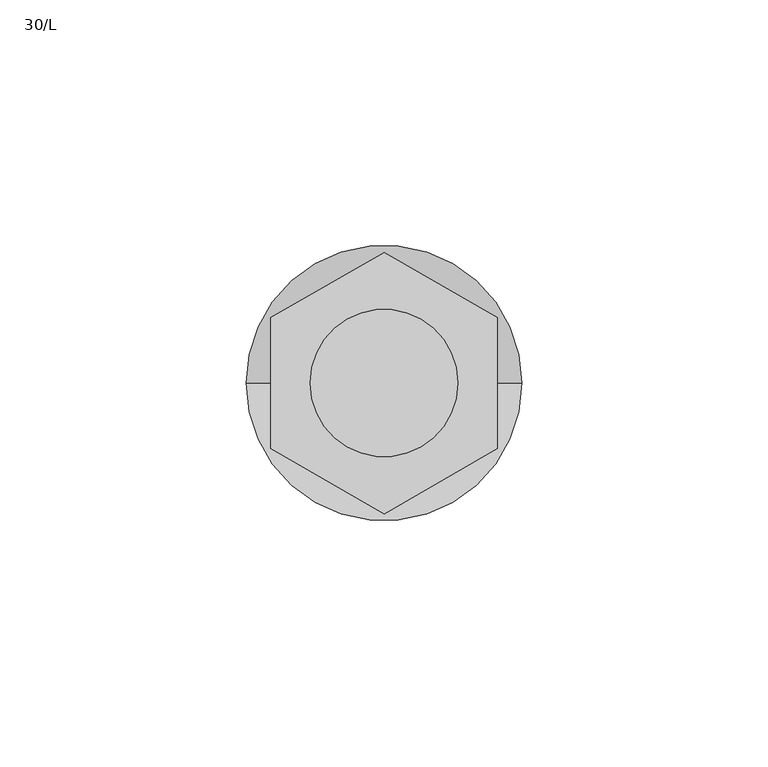
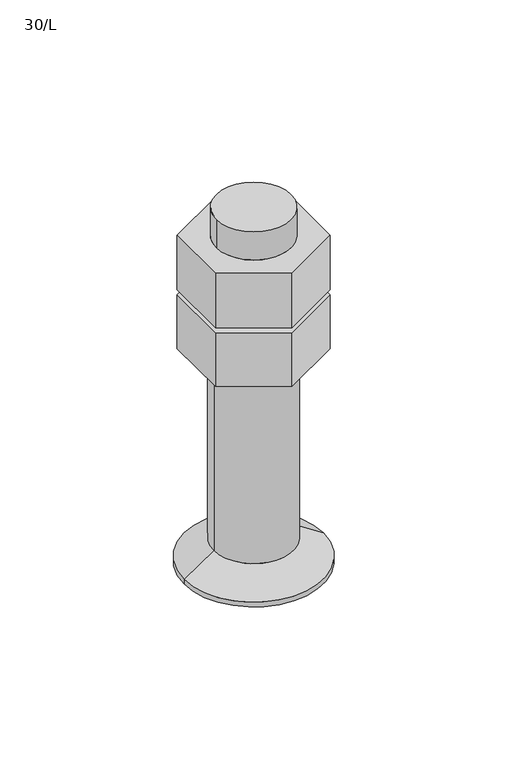
"""IFC4 building model written with IfcOpenShell, lengths in millimetres: fastener geometry, Bolt HPM-L : 30/L."""

from ifc_helpers import new_model, si_unit, frame, origin, origin_with_axes, place, context, project, spatial, polyline, circle_curve, source, transform, mapped, element, save
from ifc_brep_helpers import plane_surface, cylinder_surface, revolved_surface, advanced_brep


def fastener_30_l_d0df7ee6(model_context):
    return source(origin(), model_context, "Body", "AdvancedBrep", [
        advanced_brep(
        [(-23.0, -13.2790562, 22.7), (0.0, -26.5581124, 22.7), (23.0, -13.2790562, 22.7), (23.0, 13.2790562, 22.7), (0.0, 26.5581124, 22.7), (-23.0, 13.2790562, 22.7), (15.0, 0.0, 22.7), (-15.0, 0.0, 22.7), (-23.0, 13.2790562, 0.0), (-23.0, -13.2790562, 0.0), (0.0, 26.5581124, 0.0), (23.0, 13.2790562, 0.0), (23.0, -13.2790562, 0.0), (0.0, -26.5581124, 0.0), (-15.0, 0.0, 60.0), (15.0, 0.0, 60.0), (15.0, 0.0, 48.0), (-15.0, 0.0, 48.0), (-15.0, 0.0, 25.0), (15.0, 0.0, 25.0), (-23.0, -13.2790562, 25.0), (-23.0, 13.2790562, 25.0), (0.0, 26.5581124, 25.0), (23.0, 13.2790562, 25.0), (23.0, -13.2790562, 25.0), (0.0, -26.5581124, 25.0), (-23.0, 13.2790562, 48.0), (-23.0, -13.2790562, 48.0), (0.0, 26.5581124, 48.0), (23.0, 13.2790562, 48.0), (23.0, -13.2790562, 48.0), (0.0, -26.5581124, 48.0), (-16.0, 0.0, 0.0), (16.0, 0.0, 0.0), (16.0, 0.0, -80.0), (-16.0, 0.0, -80.0), (-28.0, 0.0, -90.0), (28.0, 0.0, -90.0), (-28.0, 0.0, -88.0), (28.0, 0.0, -88.0)],
        [
            (0, 1),
            (1, 2),
            (2, 3),
            (3, 4),
            (4, 5),
            (5, 0),
            (6, 7, circle_curve(frame((0.0, 0.0, 22.7), z_axis=(0.0, 0.0, -1.0), x_axis=(1.0, 0.0, 0.0)), 15.0)),
            (7, 6, circle_curve(frame((0.0, 0.0, 22.7), z_axis=(0.0, 0.0, -1.0), x_axis=(1.0, 0.0, 0.0)), 15.0)),
            (5, 8),
            (8, 9),
            (9, 0),
            (4, 10),
            (10, 8),
            (3, 11),
            (11, 10),
            (2, 12),
            (12, 11),
            (1, 13),
            (13, 12),
            (9, 13),
            (14, 15, circle_curve(frame((0.0, 0.0, 60.0), z_axis=(0.0, 0.0, 1.0), x_axis=(1.0, 0.0, 0.0)), 15.0)),
            (15, 14, circle_curve(frame((0.0, 0.0, 60.0), z_axis=(0.0, 0.0, 1.0), x_axis=(1.0, 0.0, 0.0)), 15.0)),
            (15, 16),
            (16, 17, circle_curve(frame((0.0, 0.0, 48.0), z_axis=(0.0, 0.0, 1.0), x_axis=(1.0, 0.0, 0.0)), 15.0)),
            (17, 14),
            (7, 18),
            (18, 19, circle_curve(frame((0.0, 0.0, 25.0), z_axis=(0.0, 0.0, -1.0), x_axis=(1.0, 0.0, 0.0)), 15.0)),
            (19, 6),
            (17, 16, circle_curve(frame((0.0, 0.0, 48.0), z_axis=(0.0, 0.0, 1.0), x_axis=(1.0, 0.0, 0.0)), 15.0)),
            (19, 18, circle_curve(frame((0.0, 0.0, 25.0), z_axis=(0.0, 0.0, -1.0), x_axis=(1.0, 0.0, 0.0)), 15.0)),
            (20, 21),
            (21, 22),
            (22, 23),
            (23, 24),
            (24, 25),
            (25, 20),
            (26, 21),
            (20, 27),
            (27, 26),
            (28, 22),
            (26, 28),
            (29, 23),
            (28, 29),
            (30, 24),
            (29, 30),
            (31, 25),
            (30, 31),
            (31, 27),
            (32, 33, circle_curve(frame((0.0, 0.0, 0.0), z_axis=(0.0, 0.0, -1.0), x_axis=(1.0, 0.0, 0.0)), 16.0)),
            (33, 34),
            (34, 35, circle_curve(frame((0.0, 0.0, -80.0), z_axis=(0.0, 0.0, 1.0), x_axis=(1.0, 0.0, 0.0)), 16.0)),
            (35, 32),
            (35, 34, circle_curve(frame((0.0, 0.0, -80.0), z_axis=(0.0, 0.0, 1.0), x_axis=(1.0, 0.0, 0.0)), 16.0)),
            (33, 32, circle_curve(frame((0.0, 0.0, 0.0), z_axis=(0.0, 0.0, -1.0), x_axis=(1.0, 0.0, 0.0)), 16.0)),
            (36, 37, circle_curve(frame((0.0, 0.0, -90.0), z_axis=(0.0, 0.0, -1.0), x_axis=(1.0, 0.0, 0.0)), 28.0)),
            (37, 36, circle_curve(frame((0.0, 0.0, -90.0), z_axis=(0.0, 0.0, -1.0), x_axis=(1.0, 0.0, 0.0)), 28.0)),
            (36, 38),
            (38, 39, circle_curve(frame((0.0, 0.0, -88.0), z_axis=(0.0, 0.0, -1.0), x_axis=(1.0, 0.0, 0.0)), 28.0)),
            (39, 37),
            (39, 38, circle_curve(frame((0.0, 0.0, -88.0), z_axis=(0.0, 0.0, -1.0), x_axis=(1.0, 0.0, 0.0)), 28.0)),
            (34, 39),
            (38, 35),
        ],
        [
            plane_surface(frame((-23.0, -13.2790562, 22.7), z_axis=(0.0, 0.0, 1.0), x_axis=(0.0, 1.0, 0.0))),
            plane_surface(frame((-23.0, -13.2790562, 22.7), z_axis=(-1.0, 0.0, 0.0), x_axis=(0.0, 0.0, -1.0))),
            plane_surface(frame((-23.0, 13.2790562, 22.7), z_axis=(-0.4999999999999993, 0.8660254037844392, 0.0), x_axis=(0.0, 0.0, -1.0))),
            plane_surface(frame((0.0, 26.5581124, 22.7), z_axis=(0.5000000000000024, 0.8660254037844374, 0.0), x_axis=(0.0, 0.0, -1.0))),
            plane_surface(frame((23.0, 13.2790562, 22.7), z_axis=(1.0, 0.0, 0.0), x_axis=(0.0, 0.0, -1.0))),
            plane_surface(frame((23.0, -13.2790562, 22.7), z_axis=(0.4999999999999989, -0.8660254037844393, 0.0), x_axis=(0.0, 0.0, -1.0))),
            plane_surface(frame((0.0, -26.5581124, 22.7), z_axis=(-0.49999999999999895, -0.8660254037844393, 0.0), x_axis=(0.0, 0.0, -1.0))),
            plane_surface(frame((15.0, 0.0, 60.0), z_axis=(0.0, 0.0, 1.0), x_axis=(0.0, -1.0, 0.0))),
            cylinder_surface(origin_with_axes(), 15.0),
            plane_surface(frame((-23.0, -13.2790562, 25.0), z_axis=(0.0, 0.0, -1.0), x_axis=(0.0, -1.0, 0.0))),
            plane_surface(frame((-23.0, -13.2790562, 48.0), z_axis=(-1.0, 0.0, 0.0), x_axis=(0.0, 0.0, -1.0))),
            plane_surface(frame((-23.0, 13.2790562, 48.0), z_axis=(-0.4999999999999995, 0.866025403784439, 0.0), x_axis=(0.0, 0.0, -1.0))),
            plane_surface(frame((0.0, 26.5581124, 48.0), z_axis=(0.5000000000000024, 0.8660254037844373, 0.0), x_axis=(0.0, 0.0, -1.0))),
            plane_surface(frame((23.0, 13.2790562, 48.0), z_axis=(1.0, 0.0, 0.0), x_axis=(0.0, 0.0, -1.0))),
            plane_surface(frame((23.0, -13.2790562, 48.0), z_axis=(0.4999999999999991, -0.8660254037844393, 0.0), x_axis=(0.0, 0.0, -1.0))),
            plane_surface(frame((0.0, -26.5581124, 48.0), z_axis=(-0.49999999999999895, -0.8660254037844393, 0.0), x_axis=(0.0, 0.0, -1.0))),
            cylinder_surface(frame((0.0, 0.0, -80.0), z_axis=(0.0, 0.0, 1.0), x_axis=(1.0, 0.0, 0.0)), 16.0),
            plane_surface(frame((28.0, 0.0, -90.0), z_axis=(0.0, 0.0, -1.0), x_axis=(0.0, 1.0, 0.0))),
            cylinder_surface(frame((0.0, 0.0, -90.0), z_axis=(0.0, 0.0, 1.0), x_axis=(1.0, 0.0, 0.0)), 28.0),
            revolved_surface(polyline([(16.00000002142857, 0.0, -80.0), (28.0, 0.0, -88.0)]), (0.0, 0.0, -69.3333333), (0.0, 0.0, -1.0)),
            revolved_surface(polyline([(-16.00000002142857, 0.0, -80.0), (-28.0, 0.0, -88.0)]), (0.0, 0.0, -69.3333333), (0.0, 0.0, -1.0)),
            plane_surface(frame((-23.0, -13.2790562, 0.0), z_axis=(0.0, 0.0, -1.0), x_axis=(0.0, -1.0, 0.0))),
            plane_surface(frame((-23.0, -13.2790562, 48.0), z_axis=(0.0, 0.0, 1.0), x_axis=(0.0, 1.0, 0.0))),
        ],
        [
            (0, [[1, 2, 3, 4, 5, 6], [7, 8]]),
            (1, [[9, 10, 11, -6]]),
            (2, [[12, 13, -9, -5]]),
            (3, [[14, 15, -12, -4]]),
            (4, [[16, 17, -14, -3]]),
            (5, [[18, 19, -16, -2]]),
            (6, [[-11, 20, -18, -1]]),
            (7, [[21, 22]]),
            (8, [[23, 24, 25, -22]]),
            (8, [[26, 27, 28, -8]]),
            (8, [[-25, 29, -23, -21]]),
            (8, [[-28, 30, -26, -7]]),
            (9, [[31, 32, 33, 34, 35, 36], [-30, -27]]),
            (10, [[37, -31, 38, 39]]),
            (11, [[40, -32, -37, 41]]),
            (12, [[42, -33, -40, 43]]),
            (13, [[44, -34, -42, 45]]),
            (14, [[46, -35, -44, 47]]),
            (15, [[-38, -36, -46, 48]]),
            (16, [[49, 50, 51, 52]]),
            (16, [[53, -50, 54, -52]]),
            (17, [[55, 56]]),
            (18, [[57, 58, 59, -55]]),
            (18, [[-59, 60, -57, -56]]),
            (19, [[-51, 61, -58, 62]]),
            (20, [[-60, -61, -53, -62]]),
            (21, [[-10, -13, -15, -17, -19, -20], [-54, -49]]),
            (22, [[-48, -47, -45, -43, -41, -39], [-29, -24]]),
        ],
    ),
    ])


if __name__ == "__main__":
    model = new_model("IFC4")
    model_context = context("Model", 3, world=origin())
    ifc_project = project(units=[si_unit("LENGTHUNIT", "METRE", prefix="MILLI")], contexts=[model_context])
    site = spatial("IfcSite", under=ifc_project)
    building = spatial("IfcBuilding", under=site)
    placement = place(None, origin())
    fastener_30_l_shape = fastener_30_l_d0df7ee6(model_context)
    element("IfcFastener", 1, ObjectType="Bolt HPM-L : 30/L", at=placement, inside=building, context=model_context, shape_type="MappedRepresentation", body=[
        mapped(fastener_30_l_shape, transform((0.0, 0.0, 0.0), x_axis=(1.0, 0.0, 0.0), y_axis=(0.0, 1.0, 0.0), z_axis=(0.0, 0.0, 1.0))),
    ])
    save(model, "model.ifc")

# Revit data of these elements
# Type "Bolt HPM-L : 30/L"
#   Type Comments = "Mountingpart"
#   r3 = 15 mm
#   r2 = 28 mm
#   r1 = 16 mm
#   offset2 = 0 mm
#   l1 = 90 mm
#   Washer s = 8 mm
#   Washer Raduis2 = 32.5 mm
#   Washer Radius1 = 15.5 mm
#   Washer Diameter2 = 65 mm
#   Washer Diameter1 = 31 mm
#   T [instance default] = 45 mm
#   Offset1 [instance default] = 25 mm
#   Hexagonal nut m = 22.7 mm
#   l3 = 60 mm
#   l2 = 90 mm
#   hef = 80 mm
#   d3 = 30 mm
#   d1 = 32 mm
#   a = 60 mm
#   Hexagonal nut S1 = 23 mm
#   Hexagonal nut S = 46 mm
#   Material [instance default] = Metal - Steel - S355
#   Default Elevation = 0
# Element 1 (IfcFastener, "Bolt HPM-L : 30/L")
#   Materials on its faces: "Metal - Steel - S355"
# Materials
#   "Metal - Steel - S355": class "Steel", colour RGB 247 247 247, transparency 0, Cost = 0
